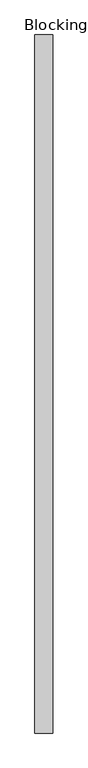
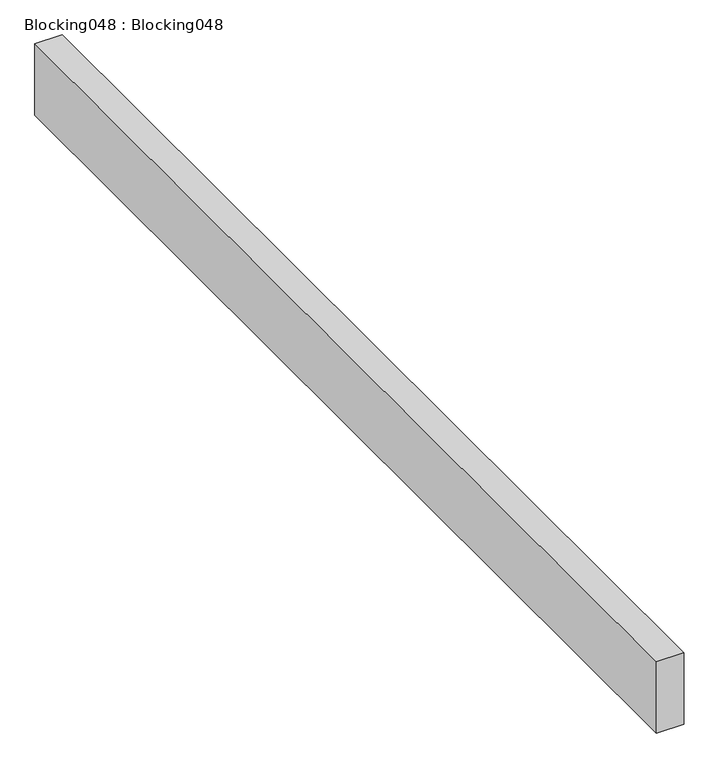
"""IFC4 building model written with IfcOpenShell, lengths in millimetres: proxy geometry, Blocking048 : Blocking048."""

import ifcopenshell
import ifcopenshell.guid

model = None  # the IFC model being written
_history = None  # IfcOwnerHistory: only IFC2X3 demands one
_inside = {}  # id of a spatial element -> (the spatial element, [elements in it])
_under = {}  # id of a project, library or spatial element -> (it, [spatial elements below it])
_declared = {}  # id of a project -> (the project, [libraries it declares])
_typed = {}  # id of a type object -> (the type object, [elements of that type])
_made_of = {}  # id of a material, layer set ... -> (it, [elements and type objects made of it])


def new_model(schema):
    """Start an empty IFC model of exactly this schema.

    Asked for "IFC4X3", IfcOpenShell would pick the latest addendum, in which some entities
    have other attributes; the version numbers below select the first issue.
    IFC2X3 requires an IfcOwnerHistory on every rooted entity: one is made here for all.
    """
    global model, _history
    if schema == "IFC4X3":
        model = ifcopenshell.file(schema_version=(4, 3, 0, 0))
    else:
        model = ifcopenshell.file(schema=schema)
    _inside.clear()
    _under.clear()
    _declared.clear()
    _typed.clear()
    _made_of.clear()
    _history = None
    if model.schema == "IFC2X3":
        org = make("IfcOrganization", Name="unknown")
        user = make(
            "IfcPersonAndOrganization",
            ThePerson=make("IfcPerson", FamilyName="unknown"),
            TheOrganization=org,
        )
        app = make(
            "IfcApplication",
            ApplicationDeveloper=org,
            Version="unknown",
            ApplicationFullName="unknown",
            ApplicationIdentifier="unknown",
        )
        _history = make(
            "IfcOwnerHistory",
            OwningUser=user,
            OwningApplication=app,
            ChangeAction="ADDED",
            CreationDate=0,
        )
    return model


def make(cls, **values):
    """One entity of the class cls with the attributes given. An attribute that is None is left unset."""
    return model.create_entity(
        cls, **{name: value for name, value in values.items() if value is not None}
    )


def rooted(cls, **values):
    """An entity with a GlobalId (a new one), such as an element, a storey or a relation."""
    return make(cls, GlobalId=ifcopenshell.guid.new(), OwnerHistory=_history, **values)


def si_unit(unit_type, name, prefix=None):
    """IfcSIUnit, for example si_unit("LENGTHUNIT", "METRE", prefix="MILLI")."""
    return make("IfcSIUnit", UnitType=unit_type, Prefix=prefix, Name=name)


def assignment(units):
    """IfcUnitAssignment: the units of a project."""
    return None if units is None else make("IfcUnitAssignment", Units=units)


def point(xyz):
    """IfcCartesianPoint."""
    return None if xyz is None else make("IfcCartesianPoint", Coordinates=xyz)


def direction(xyz):
    """IfcDirection."""
    return None if xyz is None else make("IfcDirection", DirectionRatios=xyz)


def frame(location, z_axis=None, x_axis=None):
    """IfcAxis2Placement3D, a coordinate frame: its origin and axes. An axis left out is left unset."""
    return make(
        "IfcAxis2Placement3D",
        Location=point(location),
        Axis=direction(z_axis),
        RefDirection=direction(x_axis),
    )


def origin():
    """The frame at (0, 0, 0) with its axes left unset."""
    return frame((0.0, 0.0, 0.0))


def place(relative_to, where):
    """IfcLocalPlacement: puts the frame where relative to a parent placement (None: the world)."""
    return make(
        "IfcLocalPlacement", PlacementRelTo=relative_to, RelativePlacement=where
    )


def context(
    kind, dimensions, precision=None, world=None, true_north=None, identifier=None
):
    """IfcGeometricRepresentationContext, for example the 3D "Model" context."""
    return make(
        "IfcGeometricRepresentationContext",
        ContextIdentifier=identifier,
        ContextType=kind,
        CoordinateSpaceDimension=dimensions,
        Precision=precision,
        WorldCoordinateSystem=world,
        TrueNorth=true_north,
    )


def project(units=None, contexts=None):
    """IfcProject with its units and contexts."""
    return rooted(
        "IfcProject",
        Name="project",
        RepresentationContexts=contexts,
        UnitsInContext=assignment(units),
    )


def spatial(cls, under=None, at=None, **own):
    """A site, building, storey or space (cls), placed at a placement, below another one or the project."""
    s = rooted(cls, ObjectPlacement=at, **own)
    if under is not None:
        _under.setdefault(under.id(), (under, []))[1].append(s)
    return s


def polyline(points):
    """IfcPolyline through the points."""
    return make("IfcPolyline", Points=[point(p) for p in points])


def outline(outer, holes=None, kind="AREA"):
    """IfcArbitraryClosedProfileDef: a profile drawn as a closed curve; with holes, ...WithVoids."""
    if holes is None:
        return make("IfcArbitraryClosedProfileDef", ProfileType=kind, OuterCurve=outer)
    return make(
        "IfcArbitraryProfileDefWithVoids",
        ProfileType=kind,
        OuterCurve=outer,
        InnerCurves=holes,
    )


def extrude(swept, where, along, depth):
    """IfcExtrudedAreaSolid: the profile swept, set in the frame where, extruded along a direction by depth."""
    return make(
        "IfcExtrudedAreaSolid",
        SweptArea=swept,
        Position=where,
        ExtrudedDirection=direction(along),
        Depth=depth,
    )


def shape(context_of_items, identifier, shape_type, items):
    """IfcShapeRepresentation: the items that make up one representation, for example the "Body"."""
    return make(
        "IfcShapeRepresentation",
        ContextOfItems=context_of_items,
        RepresentationIdentifier=identifier,
        RepresentationType=shape_type,
        Items=items,
    )


def source(mapping_origin, context_of_items, identifier, shape_type, items):
    """IfcRepresentationMap: a shape defined once, which mapped items show again and again."""
    return make(
        "IfcRepresentationMap",
        MappingOrigin=mapping_origin,
        MappedRepresentation=shape(context_of_items, identifier, shape_type, items),
    )


def transform(
    local_origin,
    x_axis=None,
    y_axis=None,
    z_axis=None,
    scale=None,
    scale2=None,
    scale3=None,
    uniform=True,
):
    """IfcCartesianTransformationOperator3D, or its non-uniform kind. x_axis, y_axis, z_axis: its Axis1, 2, 3."""
    if uniform:
        return make(
            "IfcCartesianTransformationOperator3D",
            Axis1=direction(x_axis),
            Axis2=direction(y_axis),
            LocalOrigin=point(local_origin),
            Scale=scale,
            Axis3=direction(z_axis),
        )
    return make(
        "IfcCartesianTransformationOperator3DnonUniform",
        Axis1=direction(x_axis),
        Axis2=direction(y_axis),
        LocalOrigin=point(local_origin),
        Scale=scale,
        Axis3=direction(z_axis),
        Scale2=scale2,
        Scale3=scale3,
    )


def mapped(mapping_source, mapping_target):
    """IfcMappedItem: shows the shape of a source again, moved by a transform."""
    return make(
        "IfcMappedItem", MappingSource=mapping_source, MappingTarget=mapping_target
    )


def made_of(thing, what):
    """Note that an element or type object is made of a material, layer set ...; save() writes the relation."""
    if what is not None:
        _made_of.setdefault(what.id(), (what, []))[1].append(thing)
    return thing


def element(
    cls,
    number,
    at=None,
    inside=None,
    cuts=None,
    type_object=None,
    material=None,
    context=None,
    identifier="Body",
    shape_type=None,
    held_by="IfcProductDefinitionShape",
    body=None,
    shapes=None,
    **own,
):
    """One element of the class cls, such as IfcWall. Its Tag is "e" and its number.

    at: its placement. inside: the storey or other place that contains it. cuts: it is an
    opening in that element (IfcRelVoidsElement). A single representation is given by context,
    identifier, shape_type and body (its items); several are given by shapes. held_by: the class
    of the entity that holds the representations. save() writes the other relations.
    """
    e = rooted(cls, Tag="e%d" % number, ObjectPlacement=at, **own)
    if body is not None:
        shapes = [shape(context, identifier, shape_type, body)]
    if shapes is not None:
        e.Representation = make(held_by, Representations=shapes)
    if inside is not None:
        _inside.setdefault(inside.id(), (inside, []))[1].append(e)
    if cuts is not None:
        rooted(
            "IfcRelVoidsElement", RelatingBuildingElement=cuts, RelatedOpeningElement=e
        )
    if type_object is not None:
        _typed.setdefault(type_object.id(), (type_object, []))[1].append(e)
    return made_of(e, material)


def aggregate(whole, parts):
    """IfcRelAggregates: a whole, such as a stair, and the parts it consists of."""
    return rooted("IfcRelAggregates", RelatingObject=whole, RelatedObjects=parts)


def save(model, path):
    """Write the relations noted so far, then the file.

    IfcRelAggregates (storeys below a building ...), IfcRelContainedInSpatialStructure (elements
    in a storey), IfcRelDefinesByType, IfcRelAssociatesMaterial and IfcRelDeclares: one each for
    every whole, place, type object, material and project.
    """
    for whole, parts in _under.values():
        aggregate(whole, parts)
    for where, things in _inside.values():
        rooted(
            "IfcRelContainedInSpatialStructure",
            RelatedElements=things,
            RelatingStructure=where,
        )
    for kind, things in _typed.values():
        rooted("IfcRelDefinesByType", RelatedObjects=things, RelatingType=kind)
    for what, things in _made_of.values():
        rooted("IfcRelAssociatesMaterial", RelatedObjects=things, RelatingMaterial=what)
    for by, libraries in _declared.values():
        rooted("IfcRelDeclares", RelatingContext=by, RelatedDefinitions=libraries)
    model.write(path)


def blocking048_blocking048_59b72ba6(model_context):
    return source(origin(), model_context, "Body", "SweptSolid", [
        extrude(outline(polyline([(-668.0864422, -1052.8908936), (-718.8864422, -1052.8908936), (-718.8864422, 947.1091064), (-668.0864422, 947.1091064), (-668.0864422, -1052.8908936)])), frame((0.0, 0.0, 39972.996), z_axis=(0.0, 0.0, 1.0), x_axis=(1.0, 0.0, 0.0)), (0.0, 0.0, 1.0), 139.7),
    ])


if __name__ == "__main__":
    model = new_model("IFC4")
    model_context = context("Model", 3, world=origin())
    ifc_project = project(units=[si_unit("LENGTHUNIT", "METRE", prefix="MILLI")], contexts=[model_context])
    site = spatial("IfcSite", under=ifc_project)
    building = spatial("IfcBuilding", under=site)
    placement = place(None, origin())
    blocking048_blocking048_shape = blocking048_blocking048_59b72ba6(model_context)
    element("IfcBuildingElementProxy", 1, Name="Blocking048 : Blocking048", ObjectType="Blocking048 : Blocking048", at=placement, inside=building, context=model_context, shape_type="MappedRepresentation", body=[
        mapped(blocking048_blocking048_shape, transform((0.0, 0.0, 0.0), x_axis=(1.0, 0.0, 0.0), y_axis=(0.0, 1.0, 0.0), z_axis=(0.0, 0.0, 1.0))),
    ])
    save(model, "model.ifc")

# Revit data of these elements
# Type "Blocking048 : Blocking048"
#   NameOverride = "Blocking048"
# Element 1 (IfcBuildingElementProxy, "Blocking048 : Blocking048")
#   Materials on its faces: "WOOD BLOCKING AS REQUIRED"
# Materials
#   "WOOD BLOCKING AS REQUIRED": class "Unassigned", colour RGB 166 124 85, transparency 0, Cost = 0
